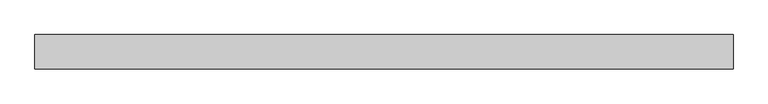
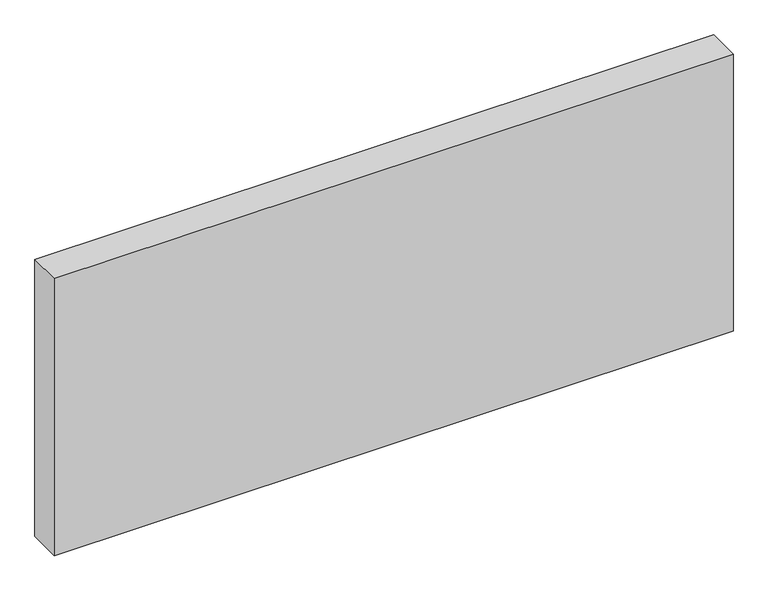
"""IFC4 building model written with IfcOpenShell, lengths in millimetres: proxy geometry, Insulation013 1163 : Insulation013 1163."""

from ifc_helpers import new_model, si_unit, frame, origin, place, context, project, spatial, polyline, outline, extrude, source, transform, mapped, element, save


def generic_models_8600da97(model_context):
    return source(origin(), model_context, "Body", "SweptSolid", [
        extrude(outline(polyline([(5694.2883192, 9716.1822682), (5694.2883192, 9617.6275807), (3694.2883192, 9617.6275807), (3694.2883192, 9716.1822682), (5694.2883192, 9716.1822682)])), frame((0.0, 0.0, 36582.0960058), z_axis=(0.0, 0.0, 1.0), x_axis=(1.0, 0.0, 0.0)), (0.0, 0.0, 1.0), 863.5993067),
    ])


if __name__ == "__main__":
    model = new_model("IFC4")
    model_context = context("Model", 3, world=origin())
    ifc_project = project(units=[si_unit("LENGTHUNIT", "METRE", prefix="MILLI")], contexts=[model_context])
    site = spatial("IfcSite", under=ifc_project)
    building = spatial("IfcBuilding", under=site)
    placement = place(None, origin())
    generic_models_shape = generic_models_8600da97(model_context)
    element("IfcBuildingElementProxy", 1, Name="Insulation013 1163 : Insulation013 1163", ObjectType="Insulation013 1163 : Insulation013 1163", at=placement, inside=building, context=model_context, shape_type="MappedRepresentation", body=[
        mapped(generic_models_shape, transform((0.0, 0.0, 0.0), x_axis=(1.0, 0.0, 0.0), y_axis=(0.0, 1.0, 0.0), z_axis=(0.0, 0.0, 1.0))),
    ])
    save(model, "model.ifc")

# Revit data of these elements
# Type "Insulation013 1163 : Insulation013 1163"
#   NameOverride = "Insulation013"
# Element 1 (IfcBuildingElementProxy, "Insulation013 1163 : Insulation013 1163")
#   Materials on its faces: "BATT INSULATION (U-FACTOR = 0.065 MIN.) OVER CLASS II VAPOR RETARDER (TOWARDS INTERIOR)"
# Materials
#   "BATT INSULATION (U-FACTOR = 0.065 MIN.) OVER CLASS II VAPOR RETARDER (TOWARDS INTERIOR)": class "Unassigned", colour RGB 246 242 160, transparency 0, Cost = 0
